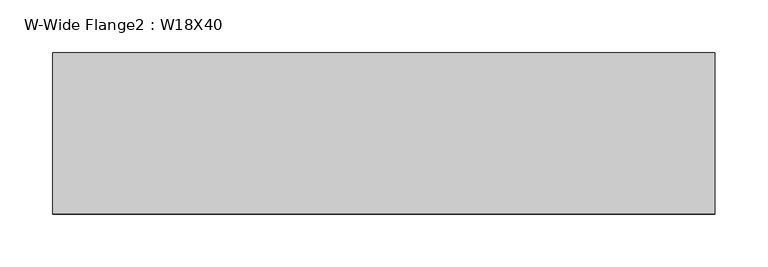
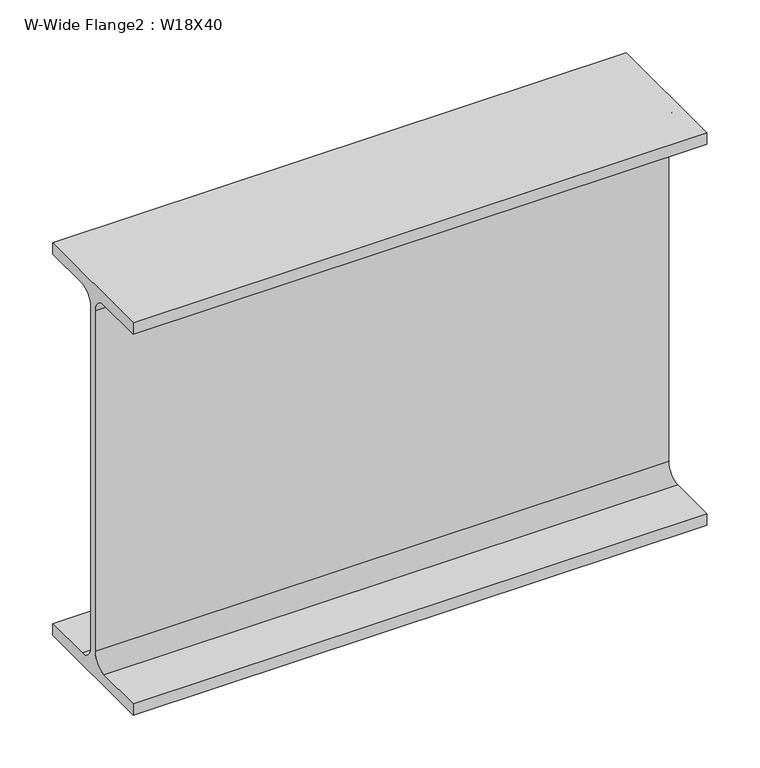
"""IFC4 building model written with IfcOpenShell, lengths in millimetres: beam geometry, W-Wide Flange2 : W18X40."""

from ifc_helpers import new_model, si_unit, point, frame, frame_2d, origin, place, context, project, spatial, polyline, circle_curve, trimmed, segment, composite_curve, outline, extrude, source, transform, mapped, element, save


def w_wide_flange2_w18x40_d42051aa(model_context):
    return source(origin(), model_context, "Body", "SweptSolid", [
        extrude(outline(composite_curve([segment(polyline([(76.454, -213.995), (76.454, -227.33), (-76.454, -227.33), (-76.454, -213.995), (-20.828, -213.995)]), True, "CONTINUOUS"), segment(trimmed(circle_curve(frame_2d((-20.828, -197.1675)), 16.8275), [point((-20.828, -213.995))], [point((-4.0005, -197.1675))], True, "CARTESIAN"), True, "CONTINUOUS"), segment(polyline([(-4.0005, -197.1675), (-4.0005, 197.1675)]), True, "CONTINUOUS"), segment(trimmed(circle_curve(frame_2d((-20.828, 197.1675)), 16.8275), [point((-4.0005, 197.1675))], [point((-20.828, 213.995))], True, "CARTESIAN"), True, "CONTINUOUS"), segment(polyline([(-20.828, 213.995), (-76.454, 213.995), (-76.454, 227.33), (76.454, 227.33), (76.454, 213.995), (20.828, 213.995)]), True, "CONTINUOUS"), segment(trimmed(circle_curve(frame_2d((20.828, 197.1675)), 16.8275), [point((20.828, 213.995))], [point((4.0005, 197.1675))], True, "CARTESIAN"), True, "CONTINUOUS"), segment(polyline([(4.0005, 197.1675), (4.0005, -197.1675)]), True, "CONTINUOUS"), segment(trimmed(circle_curve(frame_2d((20.828, -197.1675)), 16.8275), [point((4.0005, -197.1675))], [point((20.828, -213.995))], True, "CARTESIAN"), True, "CONTINUOUS"), segment(polyline([(20.828, -213.995), (76.454, -213.995)]), True, "CONTINUOUS")], self_intersect=False)), frame((-345.28125, 0.0, 0.0), z_axis=(1.0, 0.0, 0.0), x_axis=(0.0, 1.0, 0.0)), (0.0, 0.0, 1.0), 628.253125),
    ])


if __name__ == "__main__":
    model = new_model("IFC4")
    model_context = context("Model", 3, world=origin())
    ifc_project = project(units=[si_unit("LENGTHUNIT", "METRE", prefix="MILLI")], contexts=[model_context])
    site = spatial("IfcSite", under=ifc_project)
    building = spatial("IfcBuilding", under=site)
    placement = place(None, origin())
    w_wide_flange2_w18x40_shape = w_wide_flange2_w18x40_d42051aa(model_context)
    element("IfcBeam", 1, ObjectType="W-Wide Flange2 : W18X40", at=placement, inside=building, context=model_context, shape_type="MappedRepresentation", body=[
        mapped(w_wide_flange2_w18x40_shape, transform((0.0, 0.0, 0.0), x_axis=(1.0, 0.0, 0.0), y_axis=(0.0, 1.0, 0.0), z_axis=(0.0, 0.0, 1.0))),
    ])
    save(model, "model.ifc")

# Revit data of these elements
# Type "W-Wide Flange2 : W18X40"
#   Assembly Code = "B10"
#   W = 40
#   Length [instance default] = 5' - 0"
#   bf = 0' - 6.02"
#   d = 1' - 5.9"
#   k = 0' - 1 3/16"
#   k2 = 0' - 0.6625"
#   tf = 0' - 0.525"
#   tw = 0' - 0.315"
#   A = 0.0819444 SF
#   Structural Material [instance default] = Steel ASTM A992
# Element 1 (IfcBeam, "W-Wide Flange2 : W18X40")
#   Materials on its faces: "Steel ASTM A992"
# Materials
#   "Steel ASTM A992": class "Metal", colour RGB 199 199 199, transparency 0, Description = "Structural steel 50ksi", Cost = 0
